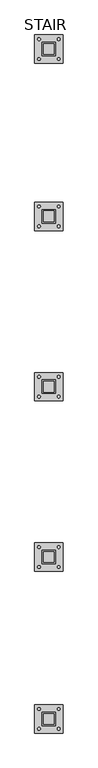
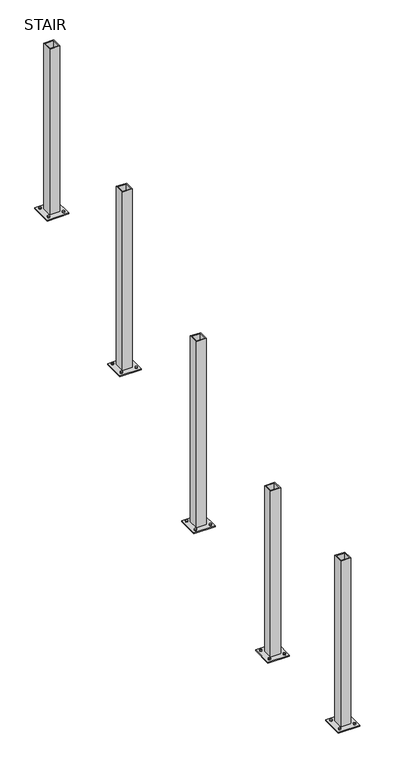
"""IFC4 building model written with IfcOpenShell, lengths in millimetres: railing geometry, STAIR."""

import ifcopenshell
import ifcopenshell.guid

model = None  # the IFC model being written
_history = None  # IfcOwnerHistory: only IFC2X3 demands one
_inside = {}  # id of a spatial element -> (the spatial element, [elements in it])
_under = {}  # id of a project, library or spatial element -> (it, [spatial elements below it])
_declared = {}  # id of a project -> (the project, [libraries it declares])
_typed = {}  # id of a type object -> (the type object, [elements of that type])
_made_of = {}  # id of a material, layer set ... -> (it, [elements and type objects made of it])


def new_model(schema):
    """Start an empty IFC model of exactly this schema.

    Asked for "IFC4X3", IfcOpenShell would pick the latest addendum, in which some entities
    have other attributes; the version numbers below select the first issue.
    IFC2X3 requires an IfcOwnerHistory on every rooted entity: one is made here for all.
    """
    global model, _history
    if schema == "IFC4X3":
        model = ifcopenshell.file(schema_version=(4, 3, 0, 0))
    else:
        model = ifcopenshell.file(schema=schema)
    _inside.clear()
    _under.clear()
    _declared.clear()
    _typed.clear()
    _made_of.clear()
    _history = None
    if model.schema == "IFC2X3":
        org = make("IfcOrganization", Name="unknown")
        user = make(
            "IfcPersonAndOrganization",
            ThePerson=make("IfcPerson", FamilyName="unknown"),
            TheOrganization=org,
        )
        app = make(
            "IfcApplication",
            ApplicationDeveloper=org,
            Version="unknown",
            ApplicationFullName="unknown",
            ApplicationIdentifier="unknown",
        )
        _history = make(
            "IfcOwnerHistory",
            OwningUser=user,
            OwningApplication=app,
            ChangeAction="ADDED",
            CreationDate=0,
        )
    return model


def make(cls, **values):
    """One entity of the class cls with the attributes given. An attribute that is None is left unset."""
    return model.create_entity(
        cls, **{name: value for name, value in values.items() if value is not None}
    )


def rooted(cls, **values):
    """An entity with a GlobalId (a new one), such as an element, a storey or a relation."""
    return make(cls, GlobalId=ifcopenshell.guid.new(), OwnerHistory=_history, **values)


def si_unit(unit_type, name, prefix=None):
    """IfcSIUnit, for example si_unit("LENGTHUNIT", "METRE", prefix="MILLI")."""
    return make("IfcSIUnit", UnitType=unit_type, Prefix=prefix, Name=name)


def assignment(units):
    """IfcUnitAssignment: the units of a project."""
    return None if units is None else make("IfcUnitAssignment", Units=units)


def point(xyz):
    """IfcCartesianPoint."""
    return None if xyz is None else make("IfcCartesianPoint", Coordinates=xyz)


def direction(xyz):
    """IfcDirection."""
    return None if xyz is None else make("IfcDirection", DirectionRatios=xyz)


def frame(location, z_axis=None, x_axis=None):
    """IfcAxis2Placement3D, a coordinate frame: its origin and axes. An axis left out is left unset."""
    return make(
        "IfcAxis2Placement3D",
        Location=point(location),
        Axis=direction(z_axis),
        RefDirection=direction(x_axis),
    )


def frame_2d(location, x_axis=None):
    """IfcAxis2Placement2D, a coordinate frame in the plane: its origin and x axis."""
    return make(
        "IfcAxis2Placement2D", Location=point(location), RefDirection=direction(x_axis)
    )


def origin():
    """The frame at (0, 0, 0) with its axes left unset."""
    return frame((0.0, 0.0, 0.0))


def place(relative_to, where):
    """IfcLocalPlacement: puts the frame where relative to a parent placement (None: the world)."""
    return make(
        "IfcLocalPlacement", PlacementRelTo=relative_to, RelativePlacement=where
    )


def context(
    kind, dimensions, precision=None, world=None, true_north=None, identifier=None
):
    """IfcGeometricRepresentationContext, for example the 3D "Model" context."""
    return make(
        "IfcGeometricRepresentationContext",
        ContextIdentifier=identifier,
        ContextType=kind,
        CoordinateSpaceDimension=dimensions,
        Precision=precision,
        WorldCoordinateSystem=world,
        TrueNorth=true_north,
    )


def project(units=None, contexts=None):
    """IfcProject with its units and contexts."""
    return rooted(
        "IfcProject",
        Name="project",
        RepresentationContexts=contexts,
        UnitsInContext=assignment(units),
    )


def spatial(cls, under=None, at=None, **own):
    """A site, building, storey or space (cls), placed at a placement, below another one or the project."""
    s = rooted(cls, ObjectPlacement=at, **own)
    if under is not None:
        _under.setdefault(under.id(), (under, []))[1].append(s)
    return s


def polyline(points):
    """IfcPolyline through the points."""
    return make("IfcPolyline", Points=[point(p) for p in points])


def circle_curve(where, radius):
    """IfcCircle in the frame where."""
    return make("IfcCircle", Position=where, Radius=radius)


def trimmed(basis, trim1, trim2, sense, master):
    """IfcTrimmedCurve: the piece of a basis curve between two trims."""
    return make(
        "IfcTrimmedCurve",
        BasisCurve=basis,
        Trim1=trim1,
        Trim2=trim2,
        SenseAgreement=sense,
        MasterRepresentation=master,
    )


def segment(curve, same_sense, transition):
    """IfcCompositeCurveSegment."""
    return make(
        "IfcCompositeCurveSegment",
        Transition=transition,
        SameSense=same_sense,
        ParentCurve=curve,
    )


def composite_curve(segments, self_intersect=None):
    """IfcCompositeCurve: segments joined end to end."""
    return make("IfcCompositeCurve", Segments=segments, SelfIntersect=self_intersect)


def outline(outer, holes=None, kind="AREA"):
    """IfcArbitraryClosedProfileDef: a profile drawn as a closed curve; with holes, ...WithVoids."""
    if holes is None:
        return make("IfcArbitraryClosedProfileDef", ProfileType=kind, OuterCurve=outer)
    return make(
        "IfcArbitraryProfileDefWithVoids",
        ProfileType=kind,
        OuterCurve=outer,
        InnerCurves=holes,
    )


def extrude(swept, where, along, depth):
    """IfcExtrudedAreaSolid: the profile swept, set in the frame where, extruded along a direction by depth."""
    return make(
        "IfcExtrudedAreaSolid",
        SweptArea=swept,
        Position=where,
        ExtrudedDirection=direction(along),
        Depth=depth,
    )


def shape(context_of_items, identifier, shape_type, items):
    """IfcShapeRepresentation: the items that make up one representation, for example the "Body"."""
    return make(
        "IfcShapeRepresentation",
        ContextOfItems=context_of_items,
        RepresentationIdentifier=identifier,
        RepresentationType=shape_type,
        Items=items,
    )


def source(mapping_origin, context_of_items, identifier, shape_type, items):
    """IfcRepresentationMap: a shape defined once, which mapped items show again and again."""
    return make(
        "IfcRepresentationMap",
        MappingOrigin=mapping_origin,
        MappedRepresentation=shape(context_of_items, identifier, shape_type, items),
    )


def transform(
    local_origin,
    x_axis=None,
    y_axis=None,
    z_axis=None,
    scale=None,
    scale2=None,
    scale3=None,
    uniform=True,
):
    """IfcCartesianTransformationOperator3D, or its non-uniform kind. x_axis, y_axis, z_axis: its Axis1, 2, 3."""
    if uniform:
        return make(
            "IfcCartesianTransformationOperator3D",
            Axis1=direction(x_axis),
            Axis2=direction(y_axis),
            LocalOrigin=point(local_origin),
            Scale=scale,
            Axis3=direction(z_axis),
        )
    return make(
        "IfcCartesianTransformationOperator3DnonUniform",
        Axis1=direction(x_axis),
        Axis2=direction(y_axis),
        LocalOrigin=point(local_origin),
        Scale=scale,
        Axis3=direction(z_axis),
        Scale2=scale2,
        Scale3=scale3,
    )


def mapped(mapping_source, mapping_target):
    """IfcMappedItem: shows the shape of a source again, moved by a transform."""
    return make(
        "IfcMappedItem", MappingSource=mapping_source, MappingTarget=mapping_target
    )


def made_of(thing, what):
    """Note that an element or type object is made of a material, layer set ...; save() writes the relation."""
    if what is not None:
        _made_of.setdefault(what.id(), (what, []))[1].append(thing)
    return thing


def element(
    cls,
    number,
    at=None,
    inside=None,
    cuts=None,
    type_object=None,
    material=None,
    context=None,
    identifier="Body",
    shape_type=None,
    held_by="IfcProductDefinitionShape",
    body=None,
    shapes=None,
    **own,
):
    """One element of the class cls, such as IfcWall. Its Tag is "e" and its number.

    at: its placement. inside: the storey or other place that contains it. cuts: it is an
    opening in that element (IfcRelVoidsElement). A single representation is given by context,
    identifier, shape_type and body (its items); several are given by shapes. held_by: the class
    of the entity that holds the representations. save() writes the other relations.
    """
    e = rooted(cls, Tag="e%d" % number, ObjectPlacement=at, **own)
    if body is not None:
        shapes = [shape(context, identifier, shape_type, body)]
    if shapes is not None:
        e.Representation = make(held_by, Representations=shapes)
    if inside is not None:
        _inside.setdefault(inside.id(), (inside, []))[1].append(e)
    if cuts is not None:
        rooted(
            "IfcRelVoidsElement", RelatingBuildingElement=cuts, RelatedOpeningElement=e
        )
    if type_object is not None:
        _typed.setdefault(type_object.id(), (type_object, []))[1].append(e)
    return made_of(e, material)


def aggregate(whole, parts):
    """IfcRelAggregates: a whole, such as a stair, and the parts it consists of."""
    return rooted("IfcRelAggregates", RelatingObject=whole, RelatedObjects=parts)


def save(model, path):
    """Write the relations noted so far, then the file.

    IfcRelAggregates (storeys below a building ...), IfcRelContainedInSpatialStructure (elements
    in a storey), IfcRelDefinesByType, IfcRelAssociatesMaterial and IfcRelDeclares: one each for
    every whole, place, type object, material and project.
    """
    for whole, parts in _under.values():
        aggregate(whole, parts)
    for where, things in _inside.values():
        rooted(
            "IfcRelContainedInSpatialStructure",
            RelatedElements=things,
            RelatingStructure=where,
        )
    for kind, things in _typed.values():
        rooted("IfcRelDefinesByType", RelatedObjects=things, RelatingType=kind)
    for what, things in _made_of.values():
        rooted("IfcRelAssociatesMaterial", RelatedObjects=things, RelatingMaterial=what)
    for by, libraries in _declared.values():
        rooted("IfcRelDeclares", RelatingContext=by, RelatedDefinitions=libraries)
    model.write(path)


def stair_c014d5bb(model_context):
    return source(origin(), model_context, "Body", "SweptSolid", [
        extrude(outline(composite_curve([segment(trimmed(circle_curve(frame_2d((26121.5120052, 5068.3543237)), 6.35), [point((26127.8620052, 5068.3543237))], [point((26115.1620052, 5068.3543237))], False, "CARTESIAN"), True, "CONTINUOUS"), segment(trimmed(circle_curve(frame_2d((26121.5120052, 5068.3543237)), 6.35), [point((26115.1620052, 5068.3543237))], [point((26127.8620052, 5068.3543237))], False, "CARTESIAN"), True, "CONTINUOUS")], self_intersect=False)), frame((0.0, 0.0, 2275.284375), z_axis=(0.0, 0.0, 1.0), x_axis=(1.0, 0.0, 0.0)), (0.0, 0.0, 1.0), 12.7),
        extrude(outline(composite_curve([segment(trimmed(circle_curve(frame_2d((26032.6120052, 5068.3543237)), 6.35), [point((26038.9620052, 5068.3543237))], [point((26026.2620052, 5068.3543237))], False, "CARTESIAN"), True, "CONTINUOUS"), segment(trimmed(circle_curve(frame_2d((26032.6120052, 5068.3543237)), 6.35), [point((26026.2620052, 5068.3543237))], [point((26038.9620052, 5068.3543237))], False, "CARTESIAN"), True, "CONTINUOUS")], self_intersect=False)), frame((0.0, 0.0, 2275.284375), z_axis=(0.0, 0.0, 1.0), x_axis=(1.0, 0.0, 0.0)), (0.0, 0.0, 1.0), 12.7),
        extrude(outline(composite_curve([segment(trimmed(circle_curve(frame_2d((26121.5120052, 5157.2543237)), 6.35), [point((26127.8620052, 5157.2543237))], [point((26115.1620052, 5157.2543237))], False, "CARTESIAN"), True, "CONTINUOUS"), segment(trimmed(circle_curve(frame_2d((26121.5120052, 5157.2543237)), 6.35), [point((26115.1620052, 5157.2543237))], [point((26127.8620052, 5157.2543237))], False, "CARTESIAN"), True, "CONTINUOUS")], self_intersect=False)), frame((0.0, 0.0, 2275.284375), z_axis=(0.0, 0.0, 1.0), x_axis=(1.0, 0.0, 0.0)), (0.0, 0.0, 1.0), 12.7),
        extrude(outline(composite_curve([segment(trimmed(circle_curve(frame_2d((26032.6120052, 5157.2543237)), 6.35), [point((26038.9620052, 5157.2543237))], [point((26026.2620052, 5157.2543237))], False, "CARTESIAN"), True, "CONTINUOUS"), segment(trimmed(circle_curve(frame_2d((26032.6120052, 5157.2543237)), 6.35), [point((26026.2620052, 5157.2543237))], [point((26038.9620052, 5157.2543237))], False, "CARTESIAN"), True, "CONTINUOUS")], self_intersect=False)), frame((0.0, 0.0, 2275.284375), z_axis=(0.0, 0.0, 1.0), x_axis=(1.0, 0.0, 0.0)), (0.0, 0.0, 1.0), 12.7),
        extrude(outline(polyline([(26013.5620052, 5049.3043237), (26013.5620052, 5176.3043237), (26140.5620052, 5176.3043237), (26140.5620052, 5049.3043237), (26013.5620052, 5049.3043237)])), frame((0.0, 0.0, 2275.284375), z_axis=(0.0, 0.0, 1.0), x_axis=(1.0, 0.0, 0.0)), (0.0, 0.0, 1.0), 6.35),
        extrude(outline(polyline([(26046.8995052, 5082.6418237), (26046.8995052, 5142.9668237), (26107.2245052, 5142.9668237), (26107.2245052, 5082.6418237), (26046.8995052, 5082.6418237)]), holes=[polyline([(26053.2495052, 5088.9918237), (26100.8745052, 5088.9918237), (26100.8745052, 5136.6168237), (26053.2495052, 5136.6168237), (26053.2495052, 5088.9918237)])]), frame((0.0, 0.0, 2275.284375), z_axis=(0.0, 0.0, 1.0), x_axis=(1.0, 0.0, 0.0)), (0.0, 0.0, 1.0), 1127.3053977),
        extrude(outline(composite_curve([segment(trimmed(circle_curve(frame_2d((26121.5120052, 4306.3543237)), 6.35), [point((26127.8620052, 4306.3543237))], [point((26115.1620052, 4306.3543237))], False, "CARTESIAN"), True, "CONTINUOUS"), segment(trimmed(circle_curve(frame_2d((26121.5120052, 4306.3543237)), 6.35), [point((26115.1620052, 4306.3543237))], [point((26127.8620052, 4306.3543237))], False, "CARTESIAN"), True, "CONTINUOUS")], self_intersect=False)), frame((0.0, 0.0, 1750.21875), z_axis=(0.0, 0.0, 1.0), x_axis=(1.0, 0.0, 0.0)), (0.0, 0.0, 1.0), 12.7),
        extrude(outline(composite_curve([segment(trimmed(circle_curve(frame_2d((26032.6120052, 4306.3543237)), 6.35), [point((26038.9620052, 4306.3543237))], [point((26026.2620052, 4306.3543237))], False, "CARTESIAN"), True, "CONTINUOUS"), segment(trimmed(circle_curve(frame_2d((26032.6120052, 4306.3543237)), 6.35), [point((26026.2620052, 4306.3543237))], [point((26038.9620052, 4306.3543237))], False, "CARTESIAN"), True, "CONTINUOUS")], self_intersect=False)), frame((0.0, 0.0, 1750.21875), z_axis=(0.0, 0.0, 1.0), x_axis=(1.0, 0.0, 0.0)), (0.0, 0.0, 1.0), 12.7),
        extrude(outline(composite_curve([segment(trimmed(circle_curve(frame_2d((26121.5120052, 4395.2543237)), 6.35), [point((26127.8620052, 4395.2543237))], [point((26115.1620052, 4395.2543237))], False, "CARTESIAN"), True, "CONTINUOUS"), segment(trimmed(circle_curve(frame_2d((26121.5120052, 4395.2543237)), 6.35), [point((26115.1620052, 4395.2543237))], [point((26127.8620052, 4395.2543237))], False, "CARTESIAN"), True, "CONTINUOUS")], self_intersect=False)), frame((0.0, 0.0, 1750.21875), z_axis=(0.0, 0.0, 1.0), x_axis=(1.0, 0.0, 0.0)), (0.0, 0.0, 1.0), 12.7),
        extrude(outline(composite_curve([segment(trimmed(circle_curve(frame_2d((26032.6120052, 4395.2543237)), 6.35), [point((26038.9620052, 4395.2543237))], [point((26026.2620052, 4395.2543237))], False, "CARTESIAN"), True, "CONTINUOUS"), segment(trimmed(circle_curve(frame_2d((26032.6120052, 4395.2543237)), 6.35), [point((26026.2620052, 4395.2543237))], [point((26038.9620052, 4395.2543237))], False, "CARTESIAN"), True, "CONTINUOUS")], self_intersect=False)), frame((0.0, 0.0, 1750.21875), z_axis=(0.0, 0.0, 1.0), x_axis=(1.0, 0.0, 0.0)), (0.0, 0.0, 1.0), 12.7),
        extrude(outline(polyline([(26013.5620052, 4287.3043237), (26013.5620052, 4414.3043237), (26140.5620052, 4414.3043237), (26140.5620052, 4287.3043237), (26013.5620052, 4287.3043237)])), frame((0.0, 0.0, 1750.21875), z_axis=(0.0, 0.0, 1.0), x_axis=(1.0, 0.0, 0.0)), (0.0, 0.0, 1.0), 6.35),
        extrude(outline(polyline([(26046.8995052, 4320.6418237), (26046.8995052, 4380.9668237), (26107.2245052, 4380.9668237), (26107.2245052, 4320.6418237), (26046.8995052, 4320.6418237)]), holes=[polyline([(26053.2495052, 4326.9918237), (26100.8745052, 4326.9918237), (26100.8745052, 4374.6168237), (26053.2495052, 4374.6168237), (26053.2495052, 4326.9918237)])]), frame((0.0, 0.0, 1750.21875), z_axis=(0.0, 0.0, 1.0), x_axis=(1.0, 0.0, 0.0)), (0.0, 0.0, 1.0), 1175.0386364),
        extrude(outline(composite_curve([segment(trimmed(circle_curve(frame_2d((26121.5120052, 3544.3543237)), 6.35), [point((26127.8620052, 3544.3543237))], [point((26115.1620052, 3544.3543237))], False, "CARTESIAN"), True, "CONTINUOUS"), segment(trimmed(circle_curve(frame_2d((26121.5120052, 3544.3543237)), 6.35), [point((26115.1620052, 3544.3543237))], [point((26127.8620052, 3544.3543237))], False, "CARTESIAN"), True, "CONTINUOUS")], self_intersect=False)), frame((0.0, 0.0, 1400.175), z_axis=(0.0, 0.0, 1.0), x_axis=(1.0, 0.0, 0.0)), (0.0, 0.0, 1.0), 12.7),
        extrude(outline(composite_curve([segment(trimmed(circle_curve(frame_2d((26032.6120052, 3544.3543237)), 6.35), [point((26038.9620052, 3544.3543237))], [point((26026.2620052, 3544.3543237))], False, "CARTESIAN"), True, "CONTINUOUS"), segment(trimmed(circle_curve(frame_2d((26032.6120052, 3544.3543237)), 6.35), [point((26026.2620052, 3544.3543237))], [point((26038.9620052, 3544.3543237))], False, "CARTESIAN"), True, "CONTINUOUS")], self_intersect=False)), frame((0.0, 0.0, 1400.175), z_axis=(0.0, 0.0, 1.0), x_axis=(1.0, 0.0, 0.0)), (0.0, 0.0, 1.0), 12.7),
        extrude(outline(composite_curve([segment(trimmed(circle_curve(frame_2d((26121.5120052, 3633.2543237)), 6.35), [point((26127.8620052, 3633.2543237))], [point((26115.1620052, 3633.2543237))], False, "CARTESIAN"), True, "CONTINUOUS"), segment(trimmed(circle_curve(frame_2d((26121.5120052, 3633.2543237)), 6.35), [point((26115.1620052, 3633.2543237))], [point((26127.8620052, 3633.2543237))], False, "CARTESIAN"), True, "CONTINUOUS")], self_intersect=False)), frame((0.0, 0.0, 1400.175), z_axis=(0.0, 0.0, 1.0), x_axis=(1.0, 0.0, 0.0)), (0.0, 0.0, 1.0), 12.7),
        extrude(outline(composite_curve([segment(trimmed(circle_curve(frame_2d((26032.6120052, 3633.2543237)), 6.35), [point((26038.9620052, 3633.2543237))], [point((26026.2620052, 3633.2543237))], False, "CARTESIAN"), True, "CONTINUOUS"), segment(trimmed(circle_curve(frame_2d((26032.6120052, 3633.2543237)), 6.35), [point((26026.2620052, 3633.2543237))], [point((26038.9620052, 3633.2543237))], False, "CARTESIAN"), True, "CONTINUOUS")], self_intersect=False)), frame((0.0, 0.0, 1400.175), z_axis=(0.0, 0.0, 1.0), x_axis=(1.0, 0.0, 0.0)), (0.0, 0.0, 1.0), 12.7),
        extrude(outline(polyline([(26013.5620052, 3525.3043237), (26013.5620052, 3652.3043237), (26140.5620052, 3652.3043237), (26140.5620052, 3525.3043237), (26013.5620052, 3525.3043237)])), frame((0.0, 0.0, 1400.175), z_axis=(0.0, 0.0, 1.0), x_axis=(1.0, 0.0, 0.0)), (0.0, 0.0, 1.0), 6.35),
        extrude(outline(polyline([(26046.8995052, 3558.6418237), (26046.8995052, 3618.9668237), (26107.2245052, 3618.9668237), (26107.2245052, 3558.6418237), (26046.8995052, 3558.6418237)]), holes=[polyline([(26053.2495052, 3564.9918237), (26100.8745052, 3564.9918237), (26100.8745052, 3612.6168237), (26053.2495052, 3612.6168237), (26053.2495052, 3564.9918237)])]), frame((0.0, 0.0, 1400.175), z_axis=(0.0, 0.0, 1.0), x_axis=(1.0, 0.0, 0.0)), (0.0, 0.0, 1.0), 1047.75),
        extrude(outline(composite_curve([segment(trimmed(circle_curve(frame_2d((26121.5120052, 5816.3134079)), 6.35), [point((26127.8620052, 5816.3134079))], [point((26115.1620052, 5816.3134079))], False, "CARTESIAN"), True, "CONTINUOUS"), segment(trimmed(circle_curve(frame_2d((26121.5120052, 5816.3134079)), 6.35), [point((26115.1620052, 5816.3134079))], [point((26127.8620052, 5816.3134079))], False, "CARTESIAN"), True, "CONTINUOUS")], self_intersect=False)), frame((0.0, 0.0, 2800.35), z_axis=(0.0, 0.0, 1.0), x_axis=(1.0, 0.0, 0.0)), (0.0, 0.0, 1.0), 12.7),
        extrude(outline(composite_curve([segment(trimmed(circle_curve(frame_2d((26032.6120052, 5816.3134079)), 6.35), [point((26038.9620052, 5816.3134079))], [point((26026.2620052, 5816.3134079))], False, "CARTESIAN"), True, "CONTINUOUS"), segment(trimmed(circle_curve(frame_2d((26032.6120052, 5816.3134079)), 6.35), [point((26026.2620052, 5816.3134079))], [point((26038.9620052, 5816.3134079))], False, "CARTESIAN"), True, "CONTINUOUS")], self_intersect=False)), frame((0.0, 0.0, 2800.35), z_axis=(0.0, 0.0, 1.0), x_axis=(1.0, 0.0, 0.0)), (0.0, 0.0, 1.0), 12.7),
        extrude(outline(composite_curve([segment(trimmed(circle_curve(frame_2d((26121.5120052, 5905.2134079)), 6.35), [point((26127.8620052, 5905.2134079))], [point((26115.1620052, 5905.2134079))], False, "CARTESIAN"), True, "CONTINUOUS"), segment(trimmed(circle_curve(frame_2d((26121.5120052, 5905.2134079)), 6.35), [point((26115.1620052, 5905.2134079))], [point((26127.8620052, 5905.2134079))], False, "CARTESIAN"), True, "CONTINUOUS")], self_intersect=False)), frame((0.0, 0.0, 2800.35), z_axis=(0.0, 0.0, 1.0), x_axis=(1.0, 0.0, 0.0)), (0.0, 0.0, 1.0), 12.7),
        extrude(outline(composite_curve([segment(trimmed(circle_curve(frame_2d((26032.6120052, 5905.2134079)), 6.35), [point((26038.9620052, 5905.2134079))], [point((26026.2620052, 5905.2134079))], False, "CARTESIAN"), True, "CONTINUOUS"), segment(trimmed(circle_curve(frame_2d((26032.6120052, 5905.2134079)), 6.35), [point((26026.2620052, 5905.2134079))], [point((26038.9620052, 5905.2134079))], False, "CARTESIAN"), True, "CONTINUOUS")], self_intersect=False)), frame((0.0, 0.0, 2800.35), z_axis=(0.0, 0.0, 1.0), x_axis=(1.0, 0.0, 0.0)), (0.0, 0.0, 1.0), 12.7),
        extrude(outline(polyline([(26013.5620052, 5797.2634079), (26013.5620052, 5924.2634079), (26140.5620052, 5924.2634079), (26140.5620052, 5797.2634079), (26013.5620052, 5797.2634079)])), frame((0.0, 0.0, 2800.35), z_axis=(0.0, 0.0, 1.0), x_axis=(1.0, 0.0, 0.0)), (0.0, 0.0, 1.0), 6.35),
        extrude(outline(polyline([(26046.8995052, 5830.6009079), (26046.8995052, 5890.9259079), (26107.2245052, 5890.9259079), (26107.2245052, 5830.6009079), (26046.8995052, 5830.6009079)]), holes=[polyline([(26053.2495052, 5836.9509079), (26100.8745052, 5836.9509079), (26100.8745052, 5884.5759079), (26053.2495052, 5884.5759079), (26053.2495052, 5836.9509079)])]), frame((0.0, 0.0, 2800.35), z_axis=(0.0, 0.0, 1.0), x_axis=(1.0, 0.0, 0.0)), (0.0, 0.0, 1.0), 1047.75),
        extrude(outline(composite_curve([segment(trimmed(circle_curve(frame_2d((26121.5120052, 2820.4543237)), 6.35), [point((26127.8620052, 2820.4543237))], [point((26115.1620052, 2820.4543237))], False, "CARTESIAN"), True, "CONTINUOUS"), segment(trimmed(circle_curve(frame_2d((26121.5120052, 2820.4543237)), 6.35), [point((26115.1620052, 2820.4543237))], [point((26127.8620052, 2820.4543237))], False, "CARTESIAN"), True, "CONTINUOUS")], self_intersect=False)), frame((0.0, 0.0, 1400.175), z_axis=(0.0, 0.0, 1.0), x_axis=(1.0, 0.0, 0.0)), (0.0, 0.0, 1.0), 12.7),
        extrude(outline(composite_curve([segment(trimmed(circle_curve(frame_2d((26032.6120052, 2820.4543237)), 6.35), [point((26038.9620052, 2820.4543237))], [point((26026.2620052, 2820.4543237))], False, "CARTESIAN"), True, "CONTINUOUS"), segment(trimmed(circle_curve(frame_2d((26032.6120052, 2820.4543237)), 6.35), [point((26026.2620052, 2820.4543237))], [point((26038.9620052, 2820.4543237))], False, "CARTESIAN"), True, "CONTINUOUS")], self_intersect=False)), frame((0.0, 0.0, 1400.175), z_axis=(0.0, 0.0, 1.0), x_axis=(1.0, 0.0, 0.0)), (0.0, 0.0, 1.0), 12.7),
        extrude(outline(composite_curve([segment(trimmed(circle_curve(frame_2d((26121.5120052, 2909.3543237)), 6.35), [point((26127.8620052, 2909.3543237))], [point((26115.1620052, 2909.3543237))], False, "CARTESIAN"), True, "CONTINUOUS"), segment(trimmed(circle_curve(frame_2d((26121.5120052, 2909.3543237)), 6.35), [point((26115.1620052, 2909.3543237))], [point((26127.8620052, 2909.3543237))], False, "CARTESIAN"), True, "CONTINUOUS")], self_intersect=False)), frame((0.0, 0.0, 1400.175), z_axis=(0.0, 0.0, 1.0), x_axis=(1.0, 0.0, 0.0)), (0.0, 0.0, 1.0), 12.7),
        extrude(outline(composite_curve([segment(trimmed(circle_curve(frame_2d((26032.6120052, 2909.3543237)), 6.35), [point((26038.9620052, 2909.3543237))], [point((26026.2620052, 2909.3543237))], False, "CARTESIAN"), True, "CONTINUOUS"), segment(trimmed(circle_curve(frame_2d((26032.6120052, 2909.3543237)), 6.35), [point((26026.2620052, 2909.3543237))], [point((26038.9620052, 2909.3543237))], False, "CARTESIAN"), True, "CONTINUOUS")], self_intersect=False)), frame((0.0, 0.0, 1400.175), z_axis=(0.0, 0.0, 1.0), x_axis=(1.0, 0.0, 0.0)), (0.0, 0.0, 1.0), 12.7),
        extrude(outline(polyline([(26013.5620052, 2801.4043237), (26013.5620052, 2928.4043237), (26140.5620052, 2928.4043237), (26140.5620052, 2801.4043237), (26013.5620052, 2801.4043237)])), frame((0.0, 0.0, 1400.175), z_axis=(0.0, 0.0, 1.0), x_axis=(1.0, 0.0, 0.0)), (0.0, 0.0, 1.0), 6.35),
        extrude(outline(polyline([(26046.8995052, 2834.7418237), (26046.8995052, 2895.0668237), (26107.2245052, 2895.0668237), (26107.2245052, 2834.7418237), (26046.8995052, 2834.7418237)]), holes=[polyline([(26053.2495052, 2841.0918237), (26100.8745052, 2841.0918237), (26100.8745052, 2888.7168237), (26053.2495052, 2888.7168237), (26053.2495052, 2841.0918237)])]), frame((0.0, 0.0, 1400.175), z_axis=(0.0, 0.0, 1.0), x_axis=(1.0, 0.0, 0.0)), (0.0, 0.0, 1.0), 1047.75),
    ])


if __name__ == "__main__":
    model = new_model("IFC4")
    model_context = context("Model", 3, world=origin())
    ifc_project = project(units=[si_unit("LENGTHUNIT", "METRE", prefix="MILLI")], contexts=[model_context])
    site = spatial("IfcSite", under=ifc_project)
    building = spatial("IfcBuilding", under=site)
    placement = place(None, origin())
    stair_shape = stair_c014d5bb(model_context)
    element("IfcRailing", 1, ObjectType="STAIR", at=placement, inside=building, context=model_context, shape_type="MappedRepresentation", body=[
        mapped(stair_shape, transform((0.0, 0.0, 0.0), x_axis=(1.0, 0.0, 0.0), y_axis=(0.0, 1.0, 0.0), z_axis=(0.0, 0.0, 1.0))),
    ])
    save(model, "model.ifc")

# Revit data of these elements
# Element 1 (IfcRailing, "STAIR")
#   Materials on its faces: "2 1/2\" X 2 1/2\" ALUM. SQUARE POST (38\" O.C. MAX)", "WIRE RAILING (3\" O.C.)", "ALUM. PLATE TOP RAIL"
# Materials
#   "2 1/2\" X 2 1/2\" ALUM. SQUARE POST (38\" O.C. MAX)": class "Metal", colour RGB 244 244 244, transparency 0, Manufacturer = "Kawneer", URL = "http://www.kawneer.com/kawneer/north_america/en/home.asp", Cost = 0
#   "WIRE RAILING (3\" O.C.)": class "Metal", colour RGB 244 244 244, transparency 0, Manufacturer = "Kawneer", URL = "http://www.kawneer.com/kawneer/north_america/en/home.asp", Cost = 0
#   "ALUM. PLATE TOP RAIL": class "Metal", colour RGB 244 244 244, transparency 0, Manufacturer = "Kawneer", URL = "http://www.kawneer.com/kawneer/north_america/en/home.asp", Cost = 0
